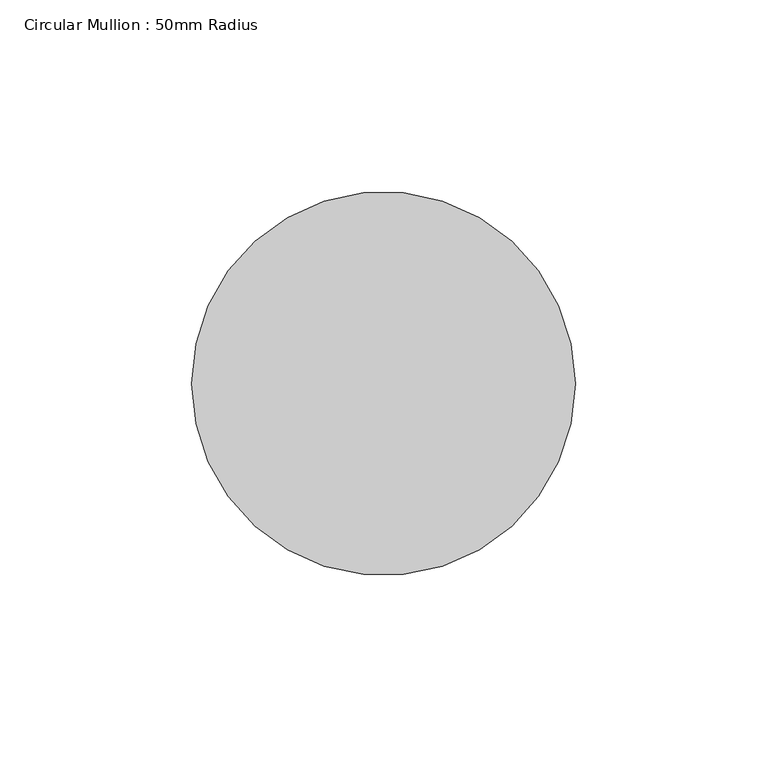
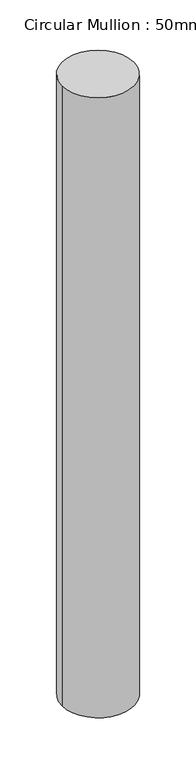
"""IFC4 building model written with IfcOpenShell, lengths in millimetres: member geometry, Circular Mullion : 50mm Radius."""

import ifcopenshell
import ifcopenshell.guid

model = None  # the IFC model being written
_history = None  # IfcOwnerHistory: only IFC2X3 demands one
_inside = {}  # id of a spatial element -> (the spatial element, [elements in it])
_under = {}  # id of a project, library or spatial element -> (it, [spatial elements below it])
_declared = {}  # id of a project -> (the project, [libraries it declares])
_typed = {}  # id of a type object -> (the type object, [elements of that type])
_made_of = {}  # id of a material, layer set ... -> (it, [elements and type objects made of it])


def new_model(schema):
    """Start an empty IFC model of exactly this schema.

    Asked for "IFC4X3", IfcOpenShell would pick the latest addendum, in which some entities
    have other attributes; the version numbers below select the first issue.
    IFC2X3 requires an IfcOwnerHistory on every rooted entity: one is made here for all.
    """
    global model, _history
    if schema == "IFC4X3":
        model = ifcopenshell.file(schema_version=(4, 3, 0, 0))
    else:
        model = ifcopenshell.file(schema=schema)
    _inside.clear()
    _under.clear()
    _declared.clear()
    _typed.clear()
    _made_of.clear()
    _history = None
    if model.schema == "IFC2X3":
        org = make("IfcOrganization", Name="unknown")
        user = make(
            "IfcPersonAndOrganization",
            ThePerson=make("IfcPerson", FamilyName="unknown"),
            TheOrganization=org,
        )
        app = make(
            "IfcApplication",
            ApplicationDeveloper=org,
            Version="unknown",
            ApplicationFullName="unknown",
            ApplicationIdentifier="unknown",
        )
        _history = make(
            "IfcOwnerHistory",
            OwningUser=user,
            OwningApplication=app,
            ChangeAction="ADDED",
            CreationDate=0,
        )
    return model


def make(cls, **values):
    """One entity of the class cls with the attributes given. An attribute that is None is left unset."""
    return model.create_entity(
        cls, **{name: value for name, value in values.items() if value is not None}
    )


def rooted(cls, **values):
    """An entity with a GlobalId (a new one), such as an element, a storey or a relation."""
    return make(cls, GlobalId=ifcopenshell.guid.new(), OwnerHistory=_history, **values)


def si_unit(unit_type, name, prefix=None):
    """IfcSIUnit, for example si_unit("LENGTHUNIT", "METRE", prefix="MILLI")."""
    return make("IfcSIUnit", UnitType=unit_type, Prefix=prefix, Name=name)


def assignment(units):
    """IfcUnitAssignment: the units of a project."""
    return None if units is None else make("IfcUnitAssignment", Units=units)


def point(xyz):
    """IfcCartesianPoint."""
    return None if xyz is None else make("IfcCartesianPoint", Coordinates=xyz)


def direction(xyz):
    """IfcDirection."""
    return None if xyz is None else make("IfcDirection", DirectionRatios=xyz)


def frame(location, z_axis=None, x_axis=None):
    """IfcAxis2Placement3D, a coordinate frame: its origin and axes. An axis left out is left unset."""
    return make(
        "IfcAxis2Placement3D",
        Location=point(location),
        Axis=direction(z_axis),
        RefDirection=direction(x_axis),
    )


def frame_2d(location, x_axis=None):
    """IfcAxis2Placement2D, a coordinate frame in the plane: its origin and x axis."""
    return make(
        "IfcAxis2Placement2D", Location=point(location), RefDirection=direction(x_axis)
    )


def origin():
    """The frame at (0, 0, 0) with its axes left unset."""
    return frame((0.0, 0.0, 0.0))


def origin_2d():
    """The frame at (0, 0) in the plane with its x axis left unset."""
    return frame_2d((0.0, 0.0))


def place(relative_to, where):
    """IfcLocalPlacement: puts the frame where relative to a parent placement (None: the world)."""
    return make(
        "IfcLocalPlacement", PlacementRelTo=relative_to, RelativePlacement=where
    )


def context(
    kind, dimensions, precision=None, world=None, true_north=None, identifier=None
):
    """IfcGeometricRepresentationContext, for example the 3D "Model" context."""
    return make(
        "IfcGeometricRepresentationContext",
        ContextIdentifier=identifier,
        ContextType=kind,
        CoordinateSpaceDimension=dimensions,
        Precision=precision,
        WorldCoordinateSystem=world,
        TrueNorth=true_north,
    )


def project(units=None, contexts=None):
    """IfcProject with its units and contexts."""
    return rooted(
        "IfcProject",
        Name="project",
        RepresentationContexts=contexts,
        UnitsInContext=assignment(units),
    )


def spatial(cls, under=None, at=None, **own):
    """A site, building, storey or space (cls), placed at a placement, below another one or the project."""
    s = rooted(cls, ObjectPlacement=at, **own)
    if under is not None:
        _under.setdefault(under.id(), (under, []))[1].append(s)
    return s


def circle_curve(where, radius):
    """IfcCircle in the frame where."""
    return make("IfcCircle", Position=where, Radius=radius)


def trimmed(basis, trim1, trim2, sense, master):
    """IfcTrimmedCurve: the piece of a basis curve between two trims."""
    return make(
        "IfcTrimmedCurve",
        BasisCurve=basis,
        Trim1=trim1,
        Trim2=trim2,
        SenseAgreement=sense,
        MasterRepresentation=master,
    )


def segment(curve, same_sense, transition):
    """IfcCompositeCurveSegment."""
    return make(
        "IfcCompositeCurveSegment",
        Transition=transition,
        SameSense=same_sense,
        ParentCurve=curve,
    )


def composite_curve(segments, self_intersect=None):
    """IfcCompositeCurve: segments joined end to end."""
    return make("IfcCompositeCurve", Segments=segments, SelfIntersect=self_intersect)


def outline(outer, holes=None, kind="AREA"):
    """IfcArbitraryClosedProfileDef: a profile drawn as a closed curve; with holes, ...WithVoids."""
    if holes is None:
        return make("IfcArbitraryClosedProfileDef", ProfileType=kind, OuterCurve=outer)
    return make(
        "IfcArbitraryProfileDefWithVoids",
        ProfileType=kind,
        OuterCurve=outer,
        InnerCurves=holes,
    )


def extrude(swept, where, along, depth):
    """IfcExtrudedAreaSolid: the profile swept, set in the frame where, extruded along a direction by depth."""
    return make(
        "IfcExtrudedAreaSolid",
        SweptArea=swept,
        Position=where,
        ExtrudedDirection=direction(along),
        Depth=depth,
    )


def shape(context_of_items, identifier, shape_type, items):
    """IfcShapeRepresentation: the items that make up one representation, for example the "Body"."""
    return make(
        "IfcShapeRepresentation",
        ContextOfItems=context_of_items,
        RepresentationIdentifier=identifier,
        RepresentationType=shape_type,
        Items=items,
    )


def source(mapping_origin, context_of_items, identifier, shape_type, items):
    """IfcRepresentationMap: a shape defined once, which mapped items show again and again."""
    return make(
        "IfcRepresentationMap",
        MappingOrigin=mapping_origin,
        MappedRepresentation=shape(context_of_items, identifier, shape_type, items),
    )


def transform(
    local_origin,
    x_axis=None,
    y_axis=None,
    z_axis=None,
    scale=None,
    scale2=None,
    scale3=None,
    uniform=True,
):
    """IfcCartesianTransformationOperator3D, or its non-uniform kind. x_axis, y_axis, z_axis: its Axis1, 2, 3."""
    if uniform:
        return make(
            "IfcCartesianTransformationOperator3D",
            Axis1=direction(x_axis),
            Axis2=direction(y_axis),
            LocalOrigin=point(local_origin),
            Scale=scale,
            Axis3=direction(z_axis),
        )
    return make(
        "IfcCartesianTransformationOperator3DnonUniform",
        Axis1=direction(x_axis),
        Axis2=direction(y_axis),
        LocalOrigin=point(local_origin),
        Scale=scale,
        Axis3=direction(z_axis),
        Scale2=scale2,
        Scale3=scale3,
    )


def mapped(mapping_source, mapping_target):
    """IfcMappedItem: shows the shape of a source again, moved by a transform."""
    return make(
        "IfcMappedItem", MappingSource=mapping_source, MappingTarget=mapping_target
    )


def made_of(thing, what):
    """Note that an element or type object is made of a material, layer set ...; save() writes the relation."""
    if what is not None:
        _made_of.setdefault(what.id(), (what, []))[1].append(thing)
    return thing


def element(
    cls,
    number,
    at=None,
    inside=None,
    cuts=None,
    type_object=None,
    material=None,
    context=None,
    identifier="Body",
    shape_type=None,
    held_by="IfcProductDefinitionShape",
    body=None,
    shapes=None,
    **own,
):
    """One element of the class cls, such as IfcWall. Its Tag is "e" and its number.

    at: its placement. inside: the storey or other place that contains it. cuts: it is an
    opening in that element (IfcRelVoidsElement). A single representation is given by context,
    identifier, shape_type and body (its items); several are given by shapes. held_by: the class
    of the entity that holds the representations. save() writes the other relations.
    """
    e = rooted(cls, Tag="e%d" % number, ObjectPlacement=at, **own)
    if body is not None:
        shapes = [shape(context, identifier, shape_type, body)]
    if shapes is not None:
        e.Representation = make(held_by, Representations=shapes)
    if inside is not None:
        _inside.setdefault(inside.id(), (inside, []))[1].append(e)
    if cuts is not None:
        rooted(
            "IfcRelVoidsElement", RelatingBuildingElement=cuts, RelatedOpeningElement=e
        )
    if type_object is not None:
        _typed.setdefault(type_object.id(), (type_object, []))[1].append(e)
    return made_of(e, material)


def aggregate(whole, parts):
    """IfcRelAggregates: a whole, such as a stair, and the parts it consists of."""
    return rooted("IfcRelAggregates", RelatingObject=whole, RelatedObjects=parts)


def save(model, path):
    """Write the relations noted so far, then the file.

    IfcRelAggregates (storeys below a building ...), IfcRelContainedInSpatialStructure (elements
    in a storey), IfcRelDefinesByType, IfcRelAssociatesMaterial and IfcRelDeclares: one each for
    every whole, place, type object, material and project.
    """
    for whole, parts in _under.values():
        aggregate(whole, parts)
    for where, things in _inside.values():
        rooted(
            "IfcRelContainedInSpatialStructure",
            RelatedElements=things,
            RelatingStructure=where,
        )
    for kind, things in _typed.values():
        rooted("IfcRelDefinesByType", RelatedObjects=things, RelatingType=kind)
    for what, things in _made_of.values():
        rooted("IfcRelAssociatesMaterial", RelatedObjects=things, RelatingMaterial=what)
    for by, libraries in _declared.values():
        rooted("IfcRelDeclares", RelatingContext=by, RelatedDefinitions=libraries)
    model.write(path)


def circular_mullion_50mm_radius_718efd37(model_context):
    return source(origin(), model_context, "Body", "SweptSolid", [
        extrude(outline(composite_curve([segment(trimmed(circle_curve(origin_2d(), 50.0), [point((50.0, 0.0))], [point((-50.0, 0.0))], False, "CARTESIAN"), True, "CONTINUOUS"), segment(trimmed(circle_curve(origin_2d(), 50.0), [point((-50.0, 0.0))], [point((50.0, 0.0))], False, "CARTESIAN"), True, "CONTINUOUS")], self_intersect=False)), frame((0.0, 0.0, -912.2982801), z_axis=(0.0, 0.0, 1.0), x_axis=(1.0, 0.0, 0.0)), (0.0, 0.0, 1.0), 912.2982801),
    ])


if __name__ == "__main__":
    model = new_model("IFC4")
    model_context = context("Model", 3, world=origin())
    ifc_project = project(units=[si_unit("LENGTHUNIT", "METRE", prefix="MILLI")], contexts=[model_context])
    site = spatial("IfcSite", under=ifc_project)
    building = spatial("IfcBuilding", under=site)
    placement = place(None, origin())
    circular_mullion_50mm_radius_shape = circular_mullion_50mm_radius_718efd37(model_context)
    element("IfcMember", 1, ObjectType="Circular Mullion : 50mm Radius", at=placement, inside=building, context=model_context, shape_type="MappedRepresentation", body=[
        mapped(circular_mullion_50mm_radius_shape, transform((0.0, 0.0, 0.0), x_axis=(1.0, 0.0, 0.0), y_axis=(0.0, 1.0, 0.0), z_axis=(0.0, 0.0, 1.0))),
    ])
    save(model, "model.ifc")

# Revit data of these elements
# Type "Circular Mullion : 50mm Radius"
#   built-in parameter 1007350 = 0.164042 (stored number, unit not read)
# Element 1 (IfcMember, "Circular Mullion : 50mm Radius")
#   Materials on its faces: "Aluminium"
# Materials
#   "Aluminium": class "Metal", colour RGB 247 247 247, transparency 0, Description = "Aluminium 6061", Cost = 0
